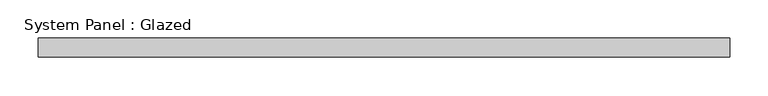
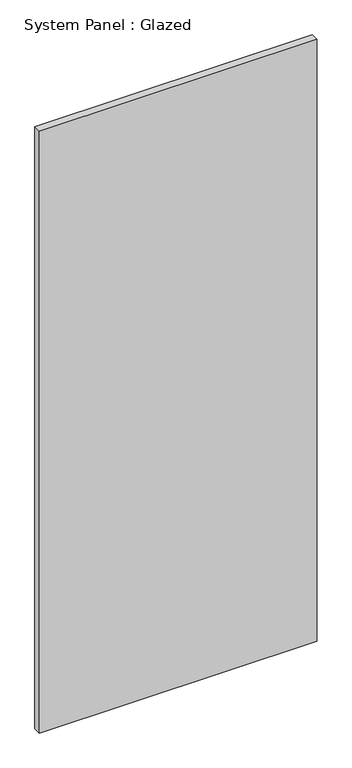
"""IFC4 building model written with IfcOpenShell, lengths in millimetres: plate geometry, System Panel : Glazed."""

from ifc_helpers import new_model, si_unit, origin, origin_with_axes, place, context, project, spatial, polyline, outline, extrude, source, transform, mapped, element, save


def system_panel_glazed_3f8cfcef(model_context):
    return source(origin(), model_context, "Body", "SweptSolid", [
        extrude(outline(polyline([(451.2500002, 24.5), (-451.2500002, 24.5), (-451.2500002, 49.5), (451.2500002, 49.5), (451.2500002, 24.5)])), origin_with_axes(), (0.0, 0.0, 1.0), 2070.0),
    ])


if __name__ == "__main__":
    model = new_model("IFC4")
    model_context = context("Model", 3, world=origin())
    ifc_project = project(units=[si_unit("LENGTHUNIT", "METRE", prefix="MILLI")], contexts=[model_context])
    site = spatial("IfcSite", under=ifc_project)
    building = spatial("IfcBuilding", under=site)
    placement = place(None, origin())
    system_panel_glazed_shape = system_panel_glazed_3f8cfcef(model_context)
    element("IfcPlate", 1, ObjectType="System Panel : Glazed", at=placement, inside=building, context=model_context, shape_type="MappedRepresentation", body=[
        mapped(system_panel_glazed_shape, transform((0.0, 0.0, 0.0), x_axis=(1.0, 0.0, 0.0), y_axis=(0.0, 1.0, 0.0), z_axis=(0.0, 0.0, 1.0))),
    ])
    save(model, "model.ifc")

# Revit data of these elements
# Type "System Panel : Glazed"
#   Construction Type Id = "GSP4R"
#   Analytic Construction = "1/8 in Pilkington single glazing"
#   Visual Light Transmittance = 0.9
#   Solar Heat Gain Coefficient = 0.86
#   Heat Transfer Coefficient (U) = 6.7069 W/(m²·K)
#   Define Thermal Properties by = 1
# Element 1 (IfcPlate, "System Panel : Glazed")
#   Materials on its faces: "Glass"
# Materials
#   "Glass": class "Glass", colour RGB 245 245 243, transparency 1, Description = "Soda Lime Glass", Cost = 0
